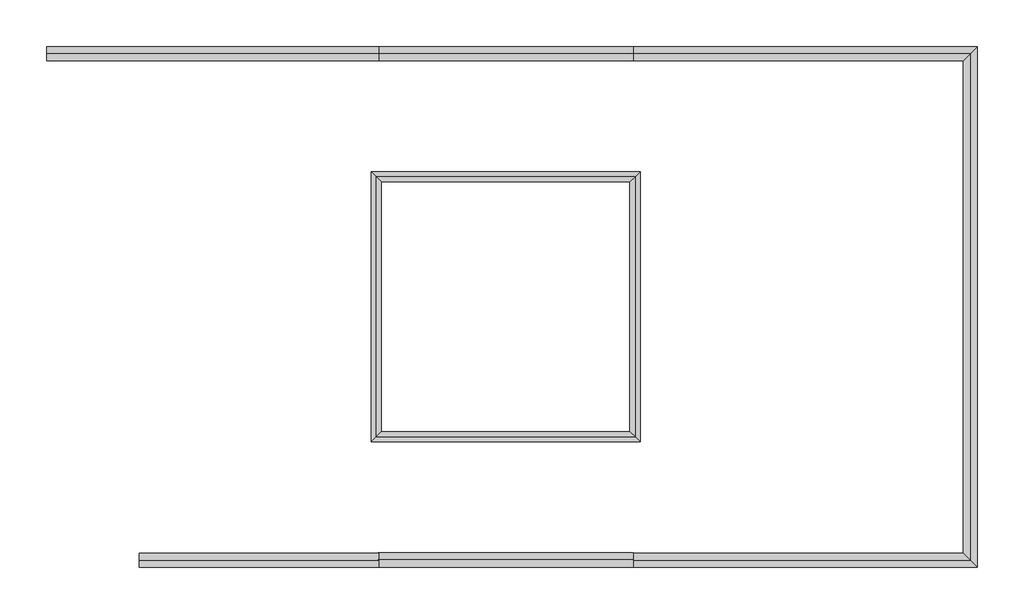
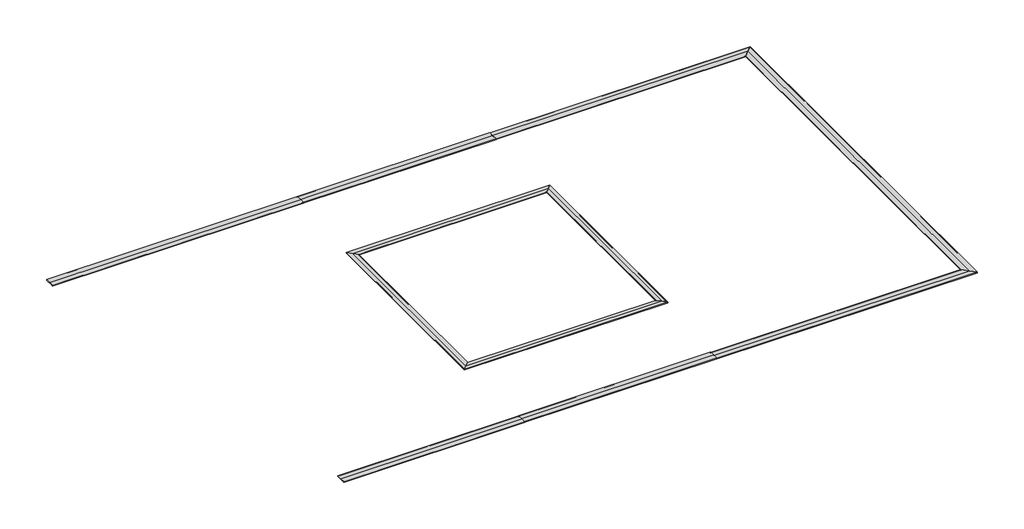
# One storey: 11 proxies.
"""IFC4 building model written with IfcOpenShell, lengths in millimetres."""

from ifc_helpers import new_model, si_unit, point, frame, frame_2d, origin, place, context, project, spatial, polyline, circle_curve, ellipse_curve, trimmed, segment, composite_curve, outline, extrude, element, save
from ifc_brep_helpers import plane_surface, revolved_surface, advanced_brep

model = new_model("IFC4")

# Units and contexts
model_context = context("Model", 3, world=origin())
ifc_project = project(units=[si_unit("LENGTHUNIT", "METRE", prefix="MILLI")], contexts=[model_context])

# Site, building, storey
site = spatial("IfcSite", under=ifc_project)
building = spatial("IfcBuilding", under=site)
storey = spatial("IfcBuildingStorey", under=building, Name="AUXILIAR-CoronacionMuro", Elevation=7150.0)

# Proxies
placement = place(None, origin())
element("IfcBuildingElementProxy", 1, Name="Wall Sweeps", at=placement, inside=storey, context=model_context, shape_type="AdvancedBrep", body=[
    advanced_brep(
    [(-12002.5, 237.5, 7180.0), (-12002.5, 237.5, 7150.0), (-12002.5, 222.6532376, 7150.0), (-12002.5, 207.6532376, 7150.0), (-12002.5, 192.5, 7150.0), (-12002.5, -217.5, 7150.0), (-12002.5, -232.6532376, 7150.0), (-12002.5, -247.6532376, 7150.0), (-12002.5, -262.5, 7150.0), (-12002.5, -262.5, 7180.0), (-12002.5, -12.5, 7184.3637662), (250.0, 237.5, 7180.0), (0.0, -12.5, 7184.3637662), (-250.0, -262.5, 7180.0), (-250.0, -262.5, 7150.0), (-235.1532376, -247.6532376, 7150.0), (-220.1532376, -232.6532376, 7150.0), (220.1532376, 207.6532376, 7150.0), (235.1532376, 222.6532376, 7150.0), (250.0, 237.5, 7150.0)],
    [
        (0, 1),
        (1, 2),
        (2, 3, circle_curve(frame((-12002.5, 215.1532376, 7150.0), z_axis=(1.0, 0.0, 0.0), x_axis=(0.0, -1.0, 0.0)), 7.5)),
        (3, 4),
        (4, 5),
        (5, 6),
        (6, 7, circle_curve(frame((-12002.5, -240.1532376, 7150.0), z_axis=(1.0, 0.0, 0.0), x_axis=(0.0, -1.0, 0.0)), 7.5)),
        (7, 8),
        (8, 9),
        (9, 10),
        (10, 0),
        (11, 12),
        (12, 13),
        (13, 14),
        (14, 15),
        (15, 16, ellipse_curve(frame((-227.6532376, -240.1532376, 7150.0), z_axis=(-0.7071067811865459, 0.7071067811865492, 0.0), x_axis=(0.707106781186549, 0.7071067811865459, 0.0)), 10.6066017, 7.5)),
        (16, 17),
        (17, 18, ellipse_curve(frame((227.6532376, 215.1532376, 7150.0), z_axis=(-0.7071067811865459, 0.7071067811865492, 0.0), x_axis=(0.707106781186549, 0.7071067811865459, 0.0)), 10.6066017, 7.5)),
        (18, 19),
        (19, 11),
        (0, 11),
        (19, 1),
        (18, 2),
        (17, 3),
        (16, 6),
        (15, 7),
        (14, 8),
        (13, 9),
        (12, 10),
    ],
    [
        plane_surface(frame((-12002.5, -217.5, 6694.0120616), z_axis=(-1.0, 0.0, 0.0), x_axis=(0.0, 1.0, 0.0))),
        plane_surface(frame((-205.0, -217.5, 7454.8), z_axis=(0.7071067811865459, -0.7071067811865492, 0.0), x_axis=(-0.7071067811865492, -0.7071067811865459, 0.0))),
        plane_surface(frame((-12002.5, 237.5, 7180.0), z_axis=(0.0, 1.0, 0.0), x_axis=(1.0, 0.0, 0.0))),
        plane_surface(frame((-12002.5, 237.5, 7150.0), z_axis=(0.0, 0.0, -1.0), x_axis=(1.0, 0.0, 0.0))),
        revolved_surface(polyline([(235.15323759999956, 207.6532376, 7150.0), (-12002.5, 207.6532376, 7150.0)]), (-12002.5, 215.1532376, 7150.0), (1.0, 0.0, 0.0)),
        plane_surface(frame((-12002.5, 207.6532376, 7150.0), z_axis=(0.0, 0.0, -1.0), x_axis=(1.0, 0.0, 0.0))),
        revolved_surface(polyline([(-220.15323759999956, -247.6532376, 7150.0), (-12002.5, -247.6532376, 7150.0)]), (-12002.5, -240.1532376, 7150.0), (1.0, 0.0, 0.0)),
        plane_surface(frame((-12002.5, -247.6532376, 7150.0), z_axis=(0.0, 0.0, -1.0), x_axis=(1.0, 0.0, 0.0))),
        plane_surface(frame((-12002.5, -262.5, 7150.0), z_axis=(0.0, -1.0, 0.0), x_axis=(1.0, 0.0, 0.0))),
        plane_surface(frame((-12002.5, -262.5, 7180.0), z_axis=(0.0, -0.017452406437287852, 0.9998476951563912), x_axis=(1.0, 0.0, 0.0))),
        plane_surface(frame((-12002.5, -12.5, 7184.3637662), z_axis=(0.0, 0.01745240643728998, 0.9998476951563912), x_axis=(1.0, 0.0, 0.0))),
    ],
    [
        (0, [[1, 2, 3, 4, 5, 6, 7, 8, 9, 10, 11]]),
        (1, [[12, 13, 14, 15, 16, 17, 18, 19, 20]]),
        (2, [[-1, 21, -20, 22]]),
        (3, [[-2, -22, -19, 23]]),
        (4, [[-3, -23, -18, 24]]),
        (5, [[-6, -5, -4, -24, -17, 25]]),
        (6, [[-7, -25, -16, 26]]),
        (7, [[-8, -26, -15, 27]]),
        (8, [[-9, -27, -14, 28]]),
        (9, [[-10, -28, -13, 29]]),
        (10, [[-11, -29, -12, -21]]),
    ],
),
])
element("IfcBuildingElementProxy", 2, Name="Wall Sweeps", at=placement, inside=storey, context=model_context, shape_type="AdvancedBrep", body=[
    advanced_brep(
    [(250.0, 237.5, 7180.0), (250.0, 237.5, 7150.0), (235.1532376, 222.6532376, 7150.0), (220.1532376, 207.6532376, 7150.0), (-220.1532376, -232.6532376, 7150.0), (-235.1532376, -247.6532376, 7150.0), (-250.0, -262.5, 7150.0), (-250.0, -262.5, 7180.0), (0.0, -12.5, 7184.3637662), (250.0, -18252.5, 7180.0), (0.0, -18002.5, 7184.3637662), (-250.0, -17752.5, 7180.0), (-250.0, -17752.5, 7150.0), (-235.1532376, -17767.3467624, 7150.0), (-220.1532376, -17782.3467624, 7150.0), (220.1532376, -18222.6532376, 7150.0), (235.1532376, -18237.6532376, 7150.0), (250.0, -18252.5, 7150.0)],
    [
        (0, 1),
        (1, 2),
        (2, 3, ellipse_curve(frame((227.6532376, 215.1532376, 7150.0), z_axis=(0.7071067811865459, -0.7071067811865492, 0.0), x_axis=(-0.7071067811865492, -0.7071067811865457, 0.0)), 10.6066017, 7.5)),
        (3, 4),
        (4, 5, ellipse_curve(frame((-227.6532376, -240.1532376, 7150.0), z_axis=(0.7071067811865459, -0.7071067811865492, 0.0), x_axis=(-0.7071067811865492, -0.7071067811865457, 0.0)), 10.6066017, 7.5)),
        (5, 6),
        (6, 7),
        (7, 8),
        (8, 0),
        (9, 10),
        (10, 11),
        (11, 12),
        (12, 13),
        (13, 14, ellipse_curve(frame((-227.6532376, -17774.8467624, 7150.0), z_axis=(0.7071067811865478, 0.7071067811865474, 0.0), x_axis=(0.7071067811865475, -0.7071067811865477, 0.0)), 10.6066017, 7.5)),
        (14, 15),
        (15, 16, ellipse_curve(frame((227.6532376, -18230.1532376, 7150.0), z_axis=(0.7071067811865478, 0.7071067811865474, 0.0), x_axis=(0.7071067811865475, -0.7071067811865477, 0.0)), 10.6066017, 7.5)),
        (16, 17),
        (17, 9),
        (0, 9),
        (17, 1),
        (16, 2),
        (15, 3),
        (14, 4),
        (13, 5),
        (12, 6),
        (11, 7),
        (10, 8),
    ],
    [
        plane_surface(frame((-205.0, -217.5, 7454.8), z_axis=(-0.7071067811865459, 0.7071067811865492, 0.0), x_axis=(-0.7071067811865492, -0.7071067811865459, 0.0))),
        plane_surface(frame((-205.0, -17797.5, 7454.8), z_axis=(-0.7071067811865478, -0.7071067811865474, 0.0), x_axis=(-0.7071067811865474, 0.7071067811865478, 0.0))),
        plane_surface(frame((250.0, 237.5, 7180.0), z_axis=(1.0, 0.0, 0.0), x_axis=(0.0, -1.0, 0.0))),
        plane_surface(frame((250.0, 237.5, 7150.0), z_axis=(0.0, 0.0, -1.0), x_axis=(0.0, -1.0, 0.0))),
        revolved_surface(polyline([(220.1532376, -18237.6532376, 7150.0), (220.1532376, 222.6532376, 7150.0)]), (227.6532376, -217.5, 7150.0), (0.0, -1.0, 0.0)),
        plane_surface(frame((220.1532376, 207.6532376, 7150.0), z_axis=(0.0, 0.0, -1.0), x_axis=(0.0, -1.0, 0.0))),
        revolved_surface(polyline([(-235.1532376, -17782.3467624, 7150.0), (-235.1532376, -232.6532376, 7150.0)]), (-227.6532376, -217.5, 7150.0), (0.0, -1.0, 0.0)),
        plane_surface(frame((-235.1532376, -247.6532376, 7150.0), z_axis=(0.0, 0.0, -1.0), x_axis=(0.0, -1.0, 0.0))),
        plane_surface(frame((-250.0, -262.5, 7150.0), z_axis=(-1.0, 0.0, 0.0), x_axis=(0.0, -1.0, 0.0))),
        plane_surface(frame((-250.0, -262.5, 7180.0), z_axis=(-0.017452406437287852, 0.0, 0.9998476951563912), x_axis=(0.0, -1.0, 0.0))),
        plane_surface(frame((0.0, -12.5, 7184.3637662), z_axis=(0.01745240643728998, 0.0, 0.9998476951563912), x_axis=(0.0, -1.0, 0.0))),
    ],
    [
        (0, [[1, 2, 3, 4, 5, 6, 7, 8, 9]]),
        (1, [[10, 11, 12, 13, 14, 15, 16, 17, 18]]),
        (2, [[-1, 19, -18, 20]]),
        (3, [[-2, -20, -17, 21]]),
        (4, [[-3, -21, -16, 22]]),
        (5, [[-4, -22, -15, 23]]),
        (6, [[-5, -23, -14, 24]]),
        (7, [[-6, -24, -13, 25]]),
        (8, [[-7, -25, -12, 26]]),
        (9, [[-8, -26, -11, 27]]),
        (10, [[-9, -27, -10, -19]]),
    ],
),
])
element("IfcBuildingElementProxy", 3, Name="Wall Sweeps", at=placement, inside=storey, context=model_context, shape_type="SweptSolid", body=[
    extrude(outline(composite_curve([segment(polyline([(237.5, 7180.0), (237.5, 7150.0), (222.6532376, 7150.0)]), True, "CONTINUOUS"), segment(trimmed(circle_curve(frame_2d((215.1532376, 7150.0)), 7.5), [point((222.6532376, 7150.0))], [point((207.6532376, 7150.0))], True, "CARTESIAN"), True, "CONTINUOUS"), segment(polyline([(207.6532376, 7150.0), (-232.6532376, 7150.0)]), True, "CONTINUOUS"), segment(trimmed(circle_curve(frame_2d((-240.1532376, 7150.0)), 7.5), [point((-232.6532376, 7150.0))], [point((-247.6532376, 7150.0))], True, "CARTESIAN"), True, "CONTINUOUS"), segment(polyline([(-247.6532376, 7150.0), (-262.5, 7150.0), (-262.5, 7180.0), (-12.5, 7184.3637662), (237.5, 7180.0)]), True, "CONTINUOUS")], self_intersect=False)), frame((-21025.0, 0.0, 0.0), z_axis=(1.0, 0.0, 0.0), x_axis=(0.0, 1.0, 0.0)), (0.0, 0.0, 1.0), 9050.0),
])
element("IfcBuildingElementProxy", 4, Name="Wall Sweeps", at=placement, inside=storey, context=model_context, shape_type="AdvancedBrep", body=[
    advanced_brep(
    [(-32795.0, 237.5, 7180.0), (-32795.0, 237.5, 7150.0), (-32795.0, 222.6532376, 7150.0), (-32795.0, 207.6532376, 7150.0), (-32795.0, -232.6532376, 7150.0), (-32795.0, -247.6532376, 7150.0), (-32795.0, -262.5, 7150.0), (-32795.0, -262.5, 7180.0), (-32795.0, -12.5, 7184.3637662), (-21010.0, 237.5, 7180.0), (-21010.0, -12.5, 7184.3637662), (-21010.0, -262.5, 7180.0), (-21010.0, -262.5, 7150.0), (-21010.0, -247.6532376, 7150.0), (-21010.0, -232.6532376, 7150.0), (-21010.0, -217.5, 7150.0), (-21010.0, 192.5, 7150.0), (-21010.0, 207.6532376, 7150.0), (-21010.0, 222.6532376, 7150.0), (-21010.0, 237.5, 7150.0)],
    [
        (0, 1),
        (1, 2),
        (2, 3, circle_curve(frame((-32795.0, 215.1532376, 7150.0), z_axis=(1.0, 0.0, 0.0), x_axis=(0.0, -1.0, 0.0)), 7.5)),
        (3, 4),
        (4, 5, circle_curve(frame((-32795.0, -240.1532376, 7150.0), z_axis=(1.0, 0.0, 0.0), x_axis=(0.0, -1.0, 0.0)), 7.5)),
        (5, 6),
        (6, 7),
        (7, 8),
        (8, 0),
        (9, 10),
        (10, 11),
        (11, 12),
        (12, 13),
        (13, 14, circle_curve(frame((-21010.0, -240.1532376, 7150.0), z_axis=(-1.0, 0.0, 0.0), x_axis=(0.0, -1.0, 0.0)), 7.5)),
        (14, 15),
        (15, 16),
        (16, 17),
        (17, 18, circle_curve(frame((-21010.0, 215.1532376, 7150.0), z_axis=(-1.0, 0.0, 0.0), x_axis=(0.0, -1.0, 0.0)), 7.5)),
        (18, 19),
        (19, 9),
        (0, 9),
        (19, 1),
        (18, 2),
        (17, 3),
        (14, 4),
        (13, 5),
        (12, 6),
        (11, 7),
        (10, 8),
    ],
    [
        plane_surface(frame((-32795.0, -217.5, 6694.0120616), z_axis=(-1.0, 0.0, 0.0), x_axis=(0.0, 1.0, 0.0))),
        plane_surface(frame((-21010.0, -217.5, 6694.0120616), z_axis=(1.0, 0.0, 0.0), x_axis=(0.0, 1.0, 0.0))),
        plane_surface(frame((-32795.0, 237.5, 7180.0), z_axis=(0.0, 1.0, 0.0), x_axis=(1.0, 0.0, 0.0))),
        plane_surface(frame((-32795.0, 237.5, 7150.0), z_axis=(0.0, 0.0, -1.0), x_axis=(1.0, 0.0, 0.0))),
        revolved_surface(polyline([(-21010.0, 207.6532376, 7150.0), (-32795.0, 207.6532376, 7150.0)]), (-32795.0, 215.1532376, 7150.0), (1.0, 0.0, 0.0)),
        plane_surface(frame((-32795.0, 207.6532376, 7150.0), z_axis=(0.0, 0.0, -1.0), x_axis=(1.0, 0.0, 0.0))),
        revolved_surface(polyline([(-21010.0, -247.6532376, 7150.0), (-32795.0, -247.6532376, 7150.0)]), (-32795.0, -240.1532376, 7150.0), (1.0, 0.0, 0.0)),
        plane_surface(frame((-32795.0, -247.6532376, 7150.0), z_axis=(0.0, 0.0, -1.0), x_axis=(1.0, 0.0, 0.0))),
        plane_surface(frame((-32795.0, -262.5, 7150.0), z_axis=(0.0, -1.0, 0.0), x_axis=(1.0, 0.0, 0.0))),
        plane_surface(frame((-32795.0, -262.5, 7180.0), z_axis=(0.0, -0.017452406437287852, 0.9998476951563912), x_axis=(1.0, 0.0, 0.0))),
        plane_surface(frame((-32795.0, -12.5, 7184.3637662), z_axis=(0.0, 0.01745240643728998, 0.9998476951563912), x_axis=(1.0, 0.0, 0.0))),
    ],
    [
        (0, [[1, 2, 3, 4, 5, 6, 7, 8, 9]]),
        (1, [[10, 11, 12, 13, 14, 15, 16, 17, 18, 19, 20]]),
        (2, [[-1, 21, -20, 22]]),
        (3, [[-2, -22, -19, 23]]),
        (4, [[-3, -23, -18, 24]]),
        (5, [[-4, -24, -17, -16, -15, 25]]),
        (6, [[-5, -25, -14, 26]]),
        (7, [[-6, -26, -13, 27]]),
        (8, [[-7, -27, -12, 28]]),
        (9, [[-8, -28, -11, 29]]),
        (10, [[-9, -29, -10, -21]]),
    ],
),
])
element("IfcBuildingElementProxy", 5, Name="Wall Sweeps", at=placement, inside=storey, context=model_context, shape_type="AdvancedBrep", body=[
    advanced_brep(
    [(250.0, -18252.5, 7180.0), (250.0, -18252.5, 7150.0), (235.1532376, -18237.6532376, 7150.0), (220.1532376, -18222.6532376, 7150.0), (-220.1532376, -17782.3467624, 7150.0), (-235.1532376, -17767.3467624, 7150.0), (-250.0, -17752.5, 7150.0), (-250.0, -17752.5, 7180.0), (0.0, -18002.5, 7184.3637662), (-11990.0, -18252.5, 7180.0), (-11990.0, -18002.5, 7184.3637662), (-11990.0, -17752.5, 7180.0), (-11990.0, -17752.5, 7150.0), (-11990.0, -17767.3467624, 7150.0), (-11990.0, -17782.3467624, 7150.0), (-11990.0, -17797.5, 7150.0), (-11990.0, -18207.5, 7150.0), (-11990.0, -18222.6532376, 7150.0), (-11990.0, -18237.6532376, 7150.0), (-11990.0, -18252.5, 7150.0)],
    [
        (0, 1),
        (1, 2),
        (2, 3, ellipse_curve(frame((227.6532376, -18230.1532376, 7150.0), z_axis=(-0.7071067811865478, -0.7071067811865474, 0.0), x_axis=(-0.7071067811865472, 0.7071067811865477, 0.0)), 10.6066017, 7.5)),
        (3, 4),
        (4, 5, ellipse_curve(frame((-227.6532376, -17774.8467624, 7150.0), z_axis=(-0.7071067811865478, -0.7071067811865474, 0.0), x_axis=(-0.7071067811865472, 0.7071067811865477, 0.0)), 10.6066017, 7.5)),
        (5, 6),
        (6, 7),
        (7, 8),
        (8, 0),
        (9, 10),
        (10, 11),
        (11, 12),
        (12, 13),
        (13, 14, circle_curve(frame((-11990.0, -17774.8467624, 7150.0), z_axis=(1.0, 0.0, 0.0), x_axis=(0.0, 1.0, 0.0)), 7.5)),
        (14, 15),
        (15, 16),
        (16, 17),
        (17, 18, circle_curve(frame((-11990.0, -18230.1532376, 7150.0), z_axis=(1.0, 0.0, 0.0), x_axis=(0.0, 1.0, 0.0)), 7.5)),
        (18, 19),
        (19, 9),
        (0, 9),
        (19, 1),
        (18, 2),
        (17, 3),
        (14, 4),
        (13, 5),
        (12, 6),
        (11, 7),
        (10, 8),
    ],
    [
        plane_surface(frame((-205.0, -17797.5, 7454.8), z_axis=(0.7071067811865478, 0.7071067811865474, 0.0), x_axis=(-0.7071067811865474, 0.7071067811865478, 0.0))),
        plane_surface(frame((-11990.0, -17797.5, 6694.0120616), z_axis=(-1.0, 0.0, 0.0), x_axis=(0.0, -1.0, 0.0))),
        plane_surface(frame((250.0, -18252.5, 7180.0), z_axis=(0.0, -1.0, 0.0), x_axis=(-1.0, 0.0, 0.0))),
        plane_surface(frame((250.0, -18252.5, 7150.0), z_axis=(0.0, 0.0, -1.0), x_axis=(-1.0, 0.0, 0.0))),
        revolved_surface(polyline([(-11990.0, -18222.6532376, 7150.0), (235.1532376, -18222.6532376, 7150.0)]), (-205.0, -18230.1532376, 7150.0), (-1.0, 0.0, 0.0)),
        plane_surface(frame((220.1532376, -18222.6532376, 7150.0), z_axis=(0.0, 0.0, -1.0), x_axis=(-1.0, 0.0, 0.0))),
        revolved_surface(polyline([(-11990.0, -17767.3467624, 7150.0), (-220.1532376, -17767.3467624, 7150.0)]), (-205.0, -17774.8467624, 7150.0), (-1.0, 0.0, 0.0)),
        plane_surface(frame((-235.1532376, -17767.3467624, 7150.0), z_axis=(0.0, 0.0, -1.0), x_axis=(-1.0, 0.0, 0.0))),
        plane_surface(frame((-250.0, -17752.5, 7150.0), z_axis=(0.0, 1.0, 0.0), x_axis=(-1.0, 0.0, 0.0))),
        plane_surface(frame((-250.0, -17752.5, 7180.0), z_axis=(0.0, 0.017452406437287852, 0.9998476951563912), x_axis=(-1.0, 0.0, 0.0))),
        plane_surface(frame((0.0, -18002.5, 7184.3637662), z_axis=(0.0, -0.01745240643728998, 0.9998476951563912), x_axis=(-1.0, 0.0, 0.0))),
    ],
    [
        (0, [[1, 2, 3, 4, 5, 6, 7, 8, 9]]),
        (1, [[10, 11, 12, 13, 14, 15, 16, 17, 18, 19, 20]]),
        (2, [[-1, 21, -20, 22]]),
        (3, [[-2, -22, -19, 23]]),
        (4, [[-3, -23, -18, 24]]),
        (5, [[-4, -24, -17, -16, -15, 25]]),
        (6, [[-5, -25, -14, 26]]),
        (7, [[-6, -26, -13, 27]]),
        (8, [[-7, -27, -12, 28]]),
        (9, [[-8, -28, -11, 29]]),
        (10, [[-9, -29, -10, -21]]),
    ],
),
])
element("IfcBuildingElementProxy", 6, Name="Wall Sweeps", at=placement, inside=storey, context=model_context, shape_type="AdvancedBrep", body=[
    advanced_brep(
    [(-21275.0, -4207.5, 7180.0), (-21275.0, -4207.5, 7150.0), (-21260.1532376, -4222.3467624, 7150.0), (-21245.1532376, -4237.3467624, 7150.0), (-20944.8467624, -4537.6532376, 7150.0), (-20929.8467624, -4552.6532376, 7150.0), (-20915.0, -4567.5, 7150.0), (-20915.0, -4567.5, 7180.0), (-21095.0, -4387.5, 7183.1419117), (-11725.0, -4207.5, 7180.0), (-11905.0, -4387.5, 7183.1419117), (-12085.0, -4567.5, 7180.0), (-12085.0, -4567.5, 7150.0), (-12070.1532376, -4552.6532376, 7150.0), (-12055.1532376, -4537.6532376, 7150.0), (-11754.8467624, -4237.3467624, 7150.0), (-11739.8467624, -4222.3467624, 7150.0), (-11725.0, -4207.5, 7150.0)],
    [
        (0, 1),
        (1, 2),
        (2, 3, ellipse_curve(frame((-21252.6532376, -4229.8467624, 7150.0), z_axis=(0.7071067811865529, 0.7071067811865422, 0.0), x_axis=(0.7071067811865421, -0.7071067811865529, 0.0)), 10.6066017, 7.5)),
        (3, 4),
        (4, 5, ellipse_curve(frame((-20937.3467624, -4545.1532376, 7150.0), z_axis=(0.7071067811865529, 0.7071067811865422, 0.0), x_axis=(0.7071067811865421, -0.7071067811865529, 0.0)), 10.6066017, 7.5)),
        (5, 6),
        (6, 7),
        (7, 8),
        (8, 0),
        (9, 10),
        (10, 11),
        (11, 12),
        (12, 13),
        (13, 14, ellipse_curve(frame((-12062.6532376, -4545.1532376, 7150.0), z_axis=(-0.7071067811865476, 0.7071067811865476, 0.0), x_axis=(0.7071067811865475, 0.7071067811865476, 0.0)), 10.6066017, 7.5)),
        (14, 15),
        (15, 16, ellipse_curve(frame((-11747.3467624, -4229.8467624, 7150.0), z_axis=(-0.7071067811865476, 0.7071067811865476, 0.0), x_axis=(0.7071067811865475, 0.7071067811865476, 0.0)), 10.6066017, 7.5)),
        (16, 17),
        (17, 9),
        (0, 9),
        (17, 1),
        (16, 2),
        (15, 3),
        (14, 4),
        (13, 5),
        (12, 6),
        (11, 7),
        (10, 8),
    ],
    [
        plane_surface(frame((-20960.0, -4522.5, 7454.8), z_axis=(-0.7071067811865529, -0.7071067811865422, 0.0), x_axis=(0.7071067811865422, -0.7071067811865529, 0.0))),
        plane_surface(frame((-12040.0, -4522.5, 7454.8), z_axis=(0.7071067811865476, -0.7071067811865476, 0.0), x_axis=(-0.7071067811865476, -0.7071067811865476, 0.0))),
        plane_surface(frame((-21275.0, -4207.5, 7180.0), z_axis=(0.0, 1.0, 0.0), x_axis=(1.0, 0.0, 0.0))),
        plane_surface(frame((-21275.0, -4207.5, 7150.0), z_axis=(0.0, 0.0, -1.0), x_axis=(1.0, 0.0, 0.0))),
        revolved_surface(polyline([(-11739.8467624, -4237.3467624, 7150.0), (-21260.1532376, -4237.3467624, 7150.0)]), (-20960.0, -4229.8467624, 7150.0), (1.0, 0.0, 0.0)),
        plane_surface(frame((-21245.1532376, -4237.3467624, 7150.0), z_axis=(0.0, 0.0, -1.0), x_axis=(1.0, 0.0, 0.0))),
        revolved_surface(polyline([(-12055.1532376, -4552.6532376, 7150.0), (-20944.8467624, -4552.6532376, 7150.0)]), (-20960.0, -4545.1532376, 7150.0), (1.0, 0.0, 0.0)),
        plane_surface(frame((-20929.8467624, -4552.6532376, 7150.0), z_axis=(0.0, 0.0, -1.0), x_axis=(1.0, 0.0, 0.0))),
        plane_surface(frame((-20915.0, -4567.5, 7150.0), z_axis=(0.0, -1.0, 0.0), x_axis=(1.0, 0.0, 0.0))),
        plane_surface(frame((-20915.0, -4567.5, 7180.0), z_axis=(0.0, -0.01745240643728671, 0.9998476951563913), x_axis=(1.0, 0.0, 0.0))),
        plane_surface(frame((-21095.0, -4387.5, 7183.1419117), z_axis=(0.0, 0.01745240643728026, 0.9998476951563914), x_axis=(1.0, 0.0, 0.0))),
    ],
    [
        (0, [[1, 2, 3, 4, 5, 6, 7, 8, 9]]),
        (1, [[10, 11, 12, 13, 14, 15, 16, 17, 18]]),
        (2, [[-1, 19, -18, 20]]),
        (3, [[-2, -20, -17, 21]]),
        (4, [[-3, -21, -16, 22]]),
        (5, [[-4, -22, -15, 23]]),
        (6, [[-5, -23, -14, 24]]),
        (7, [[-6, -24, -13, 25]]),
        (8, [[-7, -25, -12, 26]]),
        (9, [[-8, -26, -11, 27]]),
        (10, [[-9, -27, -10, -19]]),
    ],
),
])
element("IfcBuildingElementProxy", 7, Name="Wall Sweeps", at=placement, inside=storey, context=model_context, shape_type="AdvancedBrep", body=[
    advanced_brep(
    [(-11725.0, -4207.5, 7180.0), (-11725.0, -4207.5, 7150.0), (-11739.8467624, -4222.3467624, 7150.0), (-11754.8467624, -4237.3467624, 7150.0), (-12055.1532376, -4537.6532376, 7150.0), (-12070.1532376, -4552.6532376, 7150.0), (-12085.0, -4567.5, 7150.0), (-12085.0, -4567.5, 7180.0), (-11905.0, -4387.5, 7183.1419117), (-11725.0, -13792.5, 7180.0), (-11905.0, -13612.5, 7183.1419117), (-12085.0, -13432.5, 7180.0), (-12085.0, -13432.5, 7150.0), (-12070.1532376, -13447.3467624, 7150.0), (-12055.1532376, -13462.3467624, 7150.0), (-11754.8467624, -13762.6532376, 7150.0), (-11739.8467624, -13777.6532376, 7150.0), (-11725.0, -13792.5, 7150.0)],
    [
        (0, 1),
        (1, 2),
        (2, 3, ellipse_curve(frame((-11747.3467624, -4229.8467624, 7150.0), z_axis=(0.7071067811865476, -0.7071067811865476, 0.0), x_axis=(-0.7071067811865477, -0.7071067811865474, 0.0)), 10.6066017, 7.5)),
        (3, 4),
        (4, 5, ellipse_curve(frame((-12062.6532376, -4545.1532376, 7150.0), z_axis=(0.7071067811865476, -0.7071067811865476, 0.0), x_axis=(-0.7071067811865477, -0.7071067811865474, 0.0)), 10.6066017, 7.5)),
        (5, 6),
        (6, 7),
        (7, 8),
        (8, 0),
        (9, 10),
        (10, 11),
        (11, 12),
        (12, 13),
        (13, 14, ellipse_curve(frame((-12062.6532376, -13454.8467624, 7150.0), z_axis=(0.7071067811865476, 0.7071067811865476, 0.0), x_axis=(0.7071067811865477, -0.7071067811865475, 0.0)), 10.6066017, 7.5)),
        (14, 15),
        (15, 16, ellipse_curve(frame((-11747.3467624, -13770.1532376, 7150.0), z_axis=(0.7071067811865476, 0.7071067811865476, 0.0), x_axis=(0.7071067811865477, -0.7071067811865475, 0.0)), 10.6066017, 7.5)),
        (16, 17),
        (17, 9),
        (0, 9),
        (17, 1),
        (16, 2),
        (15, 3),
        (14, 4),
        (13, 5),
        (12, 6),
        (11, 7),
        (10, 8),
    ],
    [
        plane_surface(frame((-12040.0, -4522.5, 7454.8), z_axis=(-0.7071067811865476, 0.7071067811865476, 0.0), x_axis=(-0.7071067811865476, -0.7071067811865476, 0.0))),
        plane_surface(frame((-12040.0, -13477.5, 7454.8), z_axis=(-0.7071067811865476, -0.7071067811865476, 0.0), x_axis=(-0.7071067811865476, 0.7071067811865476, 0.0))),
        plane_surface(frame((-11725.0, -4207.5, 7180.0), z_axis=(1.0, 0.0, 0.0), x_axis=(0.0, -1.0, 0.0))),
        plane_surface(frame((-11725.0, -4207.5, 7150.0), z_axis=(0.0, 0.0, -1.0), x_axis=(0.0, -1.0, 0.0))),
        revolved_surface(polyline([(-11754.8467624, -13777.6532376, 7150.0), (-11754.8467624, -4222.3467624, 7150.0)]), (-11747.3467624, -4522.5, 7150.0), (0.0, -1.0, 0.0)),
        plane_surface(frame((-11754.8467624, -4237.3467624, 7150.0), z_axis=(0.0, 0.0, -1.0), x_axis=(0.0, -1.0, 0.0))),
        revolved_surface(polyline([(-12070.1532376, -13462.3467624, 7150.0), (-12070.1532376, -4537.6532376, 7150.0)]), (-12062.6532376, -4522.5, 7150.0), (0.0, -1.0, 0.0)),
        plane_surface(frame((-12070.1532376, -4552.6532376, 7150.0), z_axis=(0.0, 0.0, -1.0), x_axis=(0.0, -1.0, 0.0))),
        plane_surface(frame((-12085.0, -4567.5, 7150.0), z_axis=(-1.0, 0.0, 0.0), x_axis=(0.0, -1.0, 0.0))),
        plane_surface(frame((-12085.0, -4567.5, 7180.0), z_axis=(-0.01745240643728671, 0.0, 0.9998476951563913), x_axis=(0.0, -1.0, 0.0))),
        plane_surface(frame((-11905.0, -4387.5, 7183.1419117), z_axis=(0.01745240643728026, 0.0, 0.9998476951563914), x_axis=(0.0, -1.0, 0.0))),
    ],
    [
        (0, [[1, 2, 3, 4, 5, 6, 7, 8, 9]]),
        (1, [[10, 11, 12, 13, 14, 15, 16, 17, 18]]),
        (2, [[-1, 19, -18, 20]]),
        (3, [[-2, -20, -17, 21]]),
        (4, [[-3, -21, -16, 22]]),
        (5, [[-4, -22, -15, 23]]),
        (6, [[-5, -23, -14, 24]]),
        (7, [[-6, -24, -13, 25]]),
        (8, [[-7, -25, -12, 26]]),
        (9, [[-8, -26, -11, 27]]),
        (10, [[-9, -27, -10, -19]]),
    ],
),
])
element("IfcBuildingElementProxy", 8, Name="Wall Sweeps", at=placement, inside=storey, context=model_context, shape_type="AdvancedBrep", body=[
    advanced_brep(
    [(-11725.0, -13792.5, 7180.0), (-11725.0, -13792.5, 7150.0), (-11739.8467624, -13777.6532376, 7150.0), (-11754.8467624, -13762.6532376, 7150.0), (-12055.1532376, -13462.3467624, 7150.0), (-12070.1532376, -13447.3467624, 7150.0), (-12085.0, -13432.5, 7150.0), (-12085.0, -13432.5, 7180.0), (-11905.0, -13612.5, 7183.1419117), (-21275.0, -13792.5, 7180.0), (-21095.0, -13612.5, 7183.1419117), (-20915.0, -13432.5, 7180.0), (-20915.0, -13432.5, 7150.0), (-20929.8467624, -13447.3467624, 7150.0), (-20944.8467624, -13462.3467624, 7150.0), (-21245.1532376, -13762.6532376, 7150.0), (-21260.1532376, -13777.6532376, 7150.0), (-21275.0, -13792.5, 7150.0)],
    [
        (0, 1),
        (1, 2),
        (2, 3, ellipse_curve(frame((-11747.3467624, -13770.1532376, 7150.0), z_axis=(-0.7071067811865476, -0.7071067811865476, 0.0), x_axis=(-0.7071067811865475, 0.7071067811865476, 0.0)), 10.6066017, 7.5)),
        (3, 4),
        (4, 5, ellipse_curve(frame((-12062.6532376, -13454.8467624, 7150.0), z_axis=(-0.7071067811865476, -0.7071067811865476, 0.0), x_axis=(-0.7071067811865475, 0.7071067811865476, 0.0)), 10.6066017, 7.5)),
        (5, 6),
        (6, 7),
        (7, 8),
        (8, 0),
        (9, 10),
        (10, 11),
        (11, 12),
        (12, 13),
        (13, 14, ellipse_curve(frame((-20937.3467624, -13454.8467624, 7150.0), z_axis=(0.707106781186544, -0.7071067811865511, 0.0), x_axis=(-0.7071067811865509, -0.707106781186544, 0.0)), 10.6066017, 7.5)),
        (14, 15),
        (15, 16, ellipse_curve(frame((-21252.6532376, -13770.1532376, 7150.0), z_axis=(0.707106781186544, -0.7071067811865511, 0.0), x_axis=(-0.7071067811865509, -0.707106781186544, 0.0)), 10.6066017, 7.5)),
        (16, 17),
        (17, 9),
        (0, 9),
        (17, 1),
        (16, 2),
        (15, 3),
        (14, 4),
        (13, 5),
        (12, 6),
        (11, 7),
        (10, 8),
    ],
    [
        plane_surface(frame((-12040.0, -13477.5, 7454.8), z_axis=(0.7071067811865476, 0.7071067811865476, 0.0), x_axis=(-0.7071067811865476, 0.7071067811865476, 0.0))),
        plane_surface(frame((-20960.0, -13477.5, 7454.8), z_axis=(-0.707106781186544, 0.7071067811865511, 0.0), x_axis=(0.7071067811865511, 0.707106781186544, 0.0))),
        plane_surface(frame((-11725.0, -13792.5, 7180.0), z_axis=(0.0, -1.0, 0.0), x_axis=(-1.0, 0.0, 0.0))),
        plane_surface(frame((-11725.0, -13792.5, 7150.0), z_axis=(0.0, 0.0, -1.0), x_axis=(-1.0, 0.0, 0.0))),
        revolved_surface(polyline([(-21260.1532376, -13762.6532376, 7150.0), (-11739.8467624, -13762.6532376, 7150.0)]), (-12040.0, -13770.1532376, 7150.0), (-1.0, 0.0, 0.0)),
        plane_surface(frame((-11754.8467624, -13762.6532376, 7150.0), z_axis=(0.0, 0.0, -1.0), x_axis=(-1.0, 0.0, 0.0))),
        revolved_surface(polyline([(-20944.8467624, -13447.3467624, 7150.0), (-12055.1532376, -13447.3467624, 7150.0)]), (-12040.0, -13454.8467624, 7150.0), (-1.0, 0.0, 0.0)),
        plane_surface(frame((-12070.1532376, -13447.3467624, 7150.0), z_axis=(0.0, 0.0, -1.0), x_axis=(-1.0, 0.0, 0.0))),
        plane_surface(frame((-12085.0, -13432.5, 7150.0), z_axis=(0.0, 1.0, 0.0), x_axis=(-1.0, 0.0, 0.0))),
        plane_surface(frame((-12085.0, -13432.5, 7180.0), z_axis=(0.0, 0.01745240643728671, 0.9998476951563913), x_axis=(-1.0, 0.0, 0.0))),
        plane_surface(frame((-11905.0, -13612.5, 7183.1419117), z_axis=(0.0, -0.01745240643728026, 0.9998476951563914), x_axis=(-1.0, 0.0, 0.0))),
    ],
    [
        (0, [[1, 2, 3, 4, 5, 6, 7, 8, 9]]),
        (1, [[10, 11, 12, 13, 14, 15, 16, 17, 18]]),
        (2, [[-1, 19, -18, 20]]),
        (3, [[-2, -20, -17, 21]]),
        (4, [[-3, -21, -16, 22]]),
        (5, [[-4, -22, -15, 23]]),
        (6, [[-5, -23, -14, 24]]),
        (7, [[-6, -24, -13, 25]]),
        (8, [[-7, -25, -12, 26]]),
        (9, [[-8, -26, -11, 27]]),
        (10, [[-9, -27, -10, -19]]),
    ],
),
])
element("IfcBuildingElementProxy", 9, Name="Wall Sweeps", at=placement, inside=storey, context=model_context, shape_type="AdvancedBrep", body=[
    advanced_brep(
    [(-21275.0, -13792.5, 7180.0), (-21275.0, -13792.5, 7150.0), (-21260.1532376, -13777.6532376, 7150.0), (-21245.1532376, -13762.6532376, 7150.0), (-20944.8467624, -13462.3467624, 7150.0), (-20929.8467624, -13447.3467624, 7150.0), (-20915.0, -13432.5, 7150.0), (-20915.0, -13432.5, 7180.0), (-21095.0, -13612.5, 7183.1419117), (-21275.0, -4207.5, 7180.0), (-21095.0, -4387.5, 7183.1419117), (-20915.0, -4567.5, 7180.0), (-20915.0, -4567.5, 7150.0), (-20929.8467624, -4552.6532376, 7150.0), (-20944.8467624, -4537.6532376, 7150.0), (-21245.1532376, -4237.3467624, 7150.0), (-21260.1532376, -4222.3467624, 7150.0), (-21275.0, -4207.5, 7150.0)],
    [
        (0, 1),
        (1, 2),
        (2, 3, ellipse_curve(frame((-21252.6532376, -13770.1532376, 7150.0), z_axis=(-0.707106781186544, 0.7071067811865511, 0.0), x_axis=(0.7071067811865512, 0.7071067811865438, 0.0)), 10.6066017, 7.5)),
        (3, 4),
        (4, 5, ellipse_curve(frame((-20937.3467624, -13454.8467624, 7150.0), z_axis=(-0.707106781186544, 0.7071067811865511, 0.0), x_axis=(0.7071067811865512, 0.7071067811865438, 0.0)), 10.6066017, 7.5)),
        (5, 6),
        (6, 7),
        (7, 8),
        (8, 0),
        (9, 10),
        (10, 11),
        (11, 12),
        (12, 13),
        (13, 14, ellipse_curve(frame((-20937.3467624, -4545.1532376, 7150.0), z_axis=(-0.7071067811865529, -0.7071067811865422, 0.0), x_axis=(-0.7071067811865422, 0.7071067811865527, 0.0)), 10.6066017, 7.5)),
        (14, 15),
        (15, 16, ellipse_curve(frame((-21252.6532376, -4229.8467624, 7150.0), z_axis=(-0.7071067811865529, -0.7071067811865422, 0.0), x_axis=(-0.7071067811865422, 0.7071067811865527, 0.0)), 10.6066017, 7.5)),
        (16, 17),
        (17, 9),
        (0, 9),
        (17, 1),
        (16, 2),
        (15, 3),
        (14, 4),
        (13, 5),
        (12, 6),
        (11, 7),
        (10, 8),
    ],
    [
        plane_surface(frame((-20960.0, -13477.5, 7454.8), z_axis=(0.707106781186544, -0.7071067811865511, 0.0), x_axis=(0.7071067811865511, 0.707106781186544, 0.0))),
        plane_surface(frame((-20960.0, -4522.5, 7454.8), z_axis=(0.7071067811865529, 0.7071067811865422, 0.0), x_axis=(0.7071067811865422, -0.7071067811865529, 0.0))),
        plane_surface(frame((-21275.0, -13792.5, 7180.0), z_axis=(-1.0, 0.0, 0.0), x_axis=(0.0, 1.0, 0.0))),
        plane_surface(frame((-21275.0, -13792.5, 7150.0), z_axis=(0.0, 0.0, -1.0), x_axis=(0.0, 1.0, 0.0))),
        revolved_surface(polyline([(-21245.1532376, -4222.3467624, 7150.0), (-21245.1532376, -13777.6532376, 7150.0)]), (-21252.6532376, -13477.5, 7150.0), (0.0, 1.0, 0.0)),
        plane_surface(frame((-21245.1532376, -13762.6532376, 7150.0), z_axis=(0.0, 0.0, -1.0), x_axis=(0.0, 1.0, 0.0))),
        revolved_surface(polyline([(-20929.8467624, -4537.6532376, 7150.0), (-20929.8467624, -13462.3467624, 7150.0)]), (-20937.3467624, -13477.5, 7150.0), (0.0, 1.0, 0.0)),
        plane_surface(frame((-20929.8467624, -13447.3467624, 7150.0), z_axis=(0.0, 0.0, -1.0), x_axis=(0.0, 1.0, 0.0))),
        plane_surface(frame((-20915.0, -13432.5, 7150.0), z_axis=(1.0, 0.0, 0.0), x_axis=(0.0, 1.0, 0.0))),
        plane_surface(frame((-20915.0, -13432.5, 7180.0), z_axis=(0.01745240643728671, 0.0, 0.9998476951563913), x_axis=(0.0, 1.0, 0.0))),
        plane_surface(frame((-21095.0, -13612.5, 7183.1419117), z_axis=(-0.01745240643728026, 0.0, 0.9998476951563914), x_axis=(0.0, 1.0, 0.0))),
    ],
    [
        (0, [[1, 2, 3, 4, 5, 6, 7, 8, 9]]),
        (1, [[10, 11, 12, 13, 14, 15, 16, 17, 18]]),
        (2, [[-1, 19, -18, 20]]),
        (3, [[-2, -20, -17, 21]]),
        (4, [[-3, -21, -16, 22]]),
        (5, [[-4, -22, -15, 23]]),
        (6, [[-5, -23, -14, 24]]),
        (7, [[-6, -24, -13, 25]]),
        (8, [[-7, -25, -12, 26]]),
        (9, [[-8, -26, -11, 27]]),
        (10, [[-9, -27, -10, -19]]),
    ],
),
])
element("IfcBuildingElementProxy", 10, Name="Wall Sweeps", at=placement, inside=storey, context=model_context, shape_type="AdvancedBrep", body=[
    advanced_brep(
    [(-21010.0, -17752.5, 7180.0), (-21010.0, -18002.5, 7184.3637662), (-21010.0, -18252.5, 7180.0), (-21010.0, -18252.5, 7150.0), (-21010.0, -18237.6532376, 7150.0), (-21010.0, -18222.6532376, 7150.0), (-21010.0, -18207.5, 7150.0), (-21010.0, -17797.5, 7150.0), (-21010.0, -17782.3467624, 7150.0), (-21010.0, -17767.3467624, 7150.0), (-21010.0, -17752.5, 7150.0), (-29500.0, -17752.5, 7180.0), (-29500.0, -17752.5, 7150.0), (-29500.0, -17767.3467624, 7150.0), (-29500.0, -17782.3467624, 7150.0), (-29500.0, -17797.5, 7150.0), (-29500.0, -18207.5, 7150.0), (-29500.0, -18222.6532376, 7150.0), (-29500.0, -18237.6532376, 7150.0), (-29500.0, -18252.5, 7150.0), (-29500.0, -18252.5, 7180.0), (-29500.0, -18002.5, 7184.3637662)],
    [
        (0, 1),
        (1, 2),
        (2, 3),
        (3, 4),
        (4, 5, circle_curve(frame((-21010.0, -18230.1532376, 7150.0), z_axis=(-1.0, 0.0, 0.0), x_axis=(0.0, -1.0, 0.0)), 7.5)),
        (5, 6),
        (6, 7),
        (7, 8),
        (8, 9, circle_curve(frame((-21010.0, -17774.8467624, 7150.0), z_axis=(-1.0, 0.0, 0.0), x_axis=(0.0, -1.0, 0.0)), 7.5)),
        (9, 10),
        (10, 0),
        (11, 12),
        (12, 13),
        (13, 14, circle_curve(frame((-29500.0, -17774.8467624, 7150.0), z_axis=(1.0, 0.0, 0.0), x_axis=(0.0, -1.0, 0.0)), 7.5)),
        (14, 15),
        (15, 16),
        (16, 17),
        (17, 18, circle_curve(frame((-29500.0, -18230.1532376, 7150.0), z_axis=(1.0, 0.0, 0.0), x_axis=(0.0, -1.0, 0.0)), 7.5)),
        (18, 19),
        (19, 20),
        (20, 21),
        (21, 11),
        (0, 11),
        (21, 1),
        (20, 2),
        (19, 3),
        (18, 4),
        (17, 5),
        (14, 8),
        (13, 9),
        (12, 10),
    ],
    [
        plane_surface(frame((-21010.0, -18207.5, 6694.0120616), z_axis=(1.0, 0.0, 0.0), x_axis=(0.0, -1.0, 0.0))),
        plane_surface(frame((-29500.0, -18207.5, 6694.0120616), z_axis=(-1.0, 0.0, 0.0), x_axis=(0.0, -1.0, 0.0))),
        plane_surface(frame((-21010.0, -17752.5, 7180.0), z_axis=(0.0, 0.01745240643728998, 0.9998476951563912), x_axis=(-1.0, 0.0, 0.0))),
        plane_surface(frame((-21010.0, -18002.5, 7184.3637662), z_axis=(0.0, -0.017452406437287852, 0.9998476951563912), x_axis=(-1.0, 0.0, 0.0))),
        plane_surface(frame((-21010.0, -18252.5, 7180.0), z_axis=(0.0, -1.0, 0.0), x_axis=(-1.0, 0.0, 0.0))),
        plane_surface(frame((-21010.0, -18252.5, 7150.0), z_axis=(0.0, 0.0, -1.0), x_axis=(-1.0, 0.0, 0.0))),
        revolved_surface(polyline([(-29500.0, -18237.6532376, 7150.0), (-21010.0, -18237.6532376, 7150.0)]), (-21010.0, -18230.1532376, 7150.0), (-1.0, 0.0, 0.0)),
        plane_surface(frame((-21010.0, -18222.6532376, 7150.0), z_axis=(0.0, 0.0, -1.0), x_axis=(-1.0, 0.0, 0.0))),
        revolved_surface(polyline([(-29500.0, -17782.3467624, 7150.0), (-21010.0, -17782.3467624, 7150.0)]), (-21010.0, -17774.8467624, 7150.0), (-1.0, 0.0, 0.0)),
        plane_surface(frame((-21010.0, -17767.3467624, 7150.0), z_axis=(0.0, 0.0, -1.0), x_axis=(-1.0, 0.0, 0.0))),
        plane_surface(frame((-21010.0, -17752.5, 7150.0), z_axis=(0.0, 1.0, 0.0), x_axis=(-1.0, 0.0, 0.0))),
    ],
    [
        (0, [[1, 2, 3, 4, 5, 6, 7, 8, 9, 10, 11]]),
        (1, [[12, 13, 14, 15, 16, 17, 18, 19, 20, 21, 22]]),
        (2, [[-1, 23, -22, 24]]),
        (3, [[-2, -24, -21, 25]]),
        (4, [[-3, -25, -20, 26]]),
        (5, [[-4, -26, -19, 27]]),
        (6, [[-5, -27, -18, 28]]),
        (7, [[-8, -7, -6, -28, -17, -16, -15, 29]]),
        (8, [[-9, -29, -14, 30]]),
        (9, [[-10, -30, -13, 31]]),
        (10, [[-11, -31, -12, -23]]),
    ],
),
])
element("IfcBuildingElementProxy", 11, Name="Wall Sweeps", at=placement, inside=storey, context=model_context, shape_type="SweptSolid", body=[
    extrude(outline(composite_curve([segment(polyline([(-17737.5, 7180.0), (-17737.5, 7150.0), (-17752.3467624, 7150.0)]), True, "CONTINUOUS"), segment(trimmed(circle_curve(frame_2d((-17759.8467624, 7150.0)), 7.5), [point((-17752.3467624, 7150.0))], [point((-17767.3467624, 7150.0))], True, "CARTESIAN"), True, "CONTINUOUS"), segment(polyline([(-17767.3467624, 7150.0), (-18207.6532376, 7150.0)]), True, "CONTINUOUS"), segment(trimmed(circle_curve(frame_2d((-18215.1532376, 7150.0)), 7.5), [point((-18207.6532376, 7150.0))], [point((-18222.6532376, 7150.0))], True, "CARTESIAN"), True, "CONTINUOUS"), segment(polyline([(-18222.6532376, 7150.0), (-18237.5, 7150.0), (-18237.5, 7180.0), (-17987.5, 7184.3637662), (-17737.5, 7180.0)]), True, "CONTINUOUS")], self_intersect=False)), frame((-21025.0, 0.0, 0.0), z_axis=(1.0, 0.0, 0.0), x_axis=(0.0, 1.0, 0.0)), (0.0, 0.0, 1.0), 9050.0),
])

save(model, "model.ifc")

# Revit data of these elements
# Elements 1, 2, 3, 4, 5, 6, 7, 8, 9, 10, 11 (IfcBuildingElementProxy)
#   Phase Created = Nueva construcción
#   Materials on its faces: "Muro por defecto"
# Materials
#   "Muro por defecto": class "Varios", colour RGB 212 212 212, transparency 0, Cost = 0
